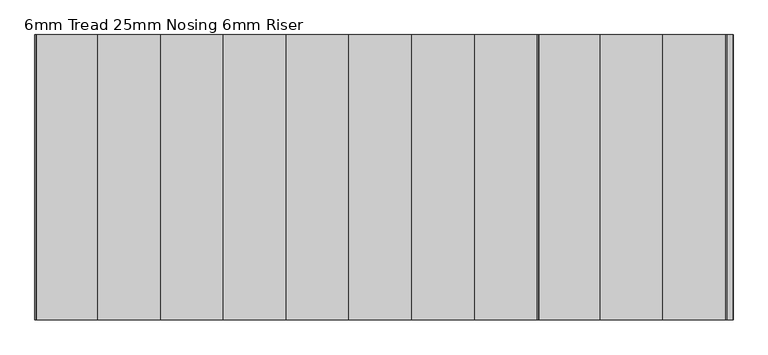
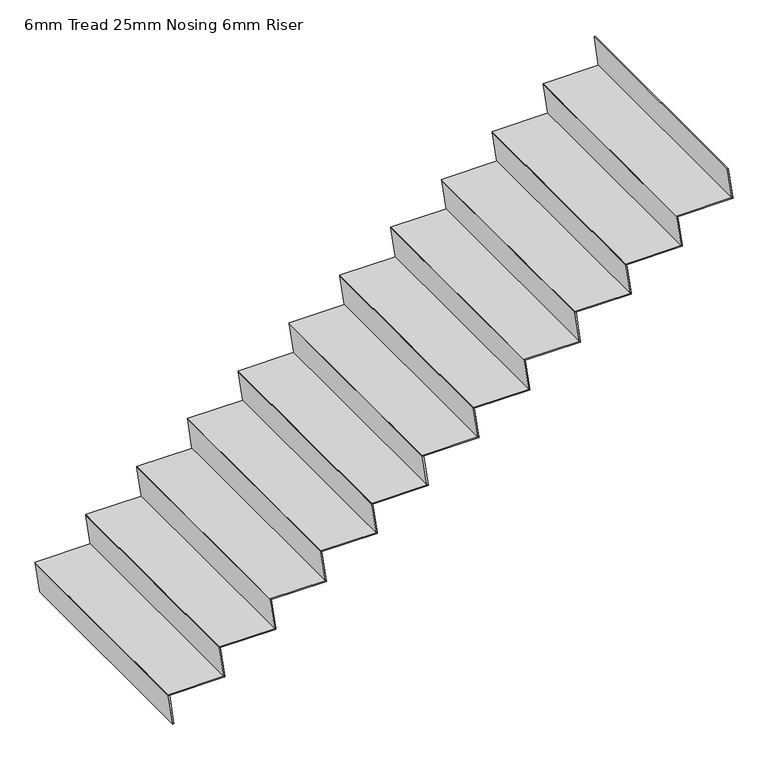
"""IFC4 building model written with IfcOpenShell, lengths in millimetres: stair flight geometry, 6mm Tread 25mm Nosing 6mm Riser."""

from ifc_helpers import new_model, si_unit, frame, origin, place, context, project, spatial, polyline, outline, extrude, source, transform, mapped, element, save


def stair_flight_6mm_tread_25mm_nosing_6mm_riser_570a7bc1(model_context):
    return source(origin(), model_context, "Body", "SweptSolid", [
        extrude(outline(polyline([(4266.6666667, 13631.0590357), (4266.6666667, 13325.0), (4260.6666667, 13325.84375), (4260.6666667, 13631.9027857), (4266.6666667, 13631.0590357)])), frame((0.0, 10220.4345331, 0.0), z_axis=(0.0, 1.0, 0.0), x_axis=(0.0, 0.0, 1.0)), (0.0, 0.0, 1.0), 1250.0),
        extrude(outline(polyline([(4260.6666667, 13325.84375), (4088.8888889, 13350.0), (4088.8888889, 13356.0590357), (4260.6666667, 13331.9027857), (4260.6666667, 13325.84375)])), frame((0.0, 10220.4345331, 0.0), z_axis=(0.0, 1.0, 0.0), x_axis=(0.0, 0.0, 1.0)), (0.0, 0.0, 1.0), 1250.0),
        extrude(outline(polyline([(4438.4444444, 13600.84375), (4266.6666667, 13625.0), (4266.6666667, 13631.0590357), (4438.4444444, 13606.9027857), (4438.4444444, 13600.84375)])), frame((0.0, 10220.4345331, 0.0), z_axis=(0.0, 1.0, 0.0), x_axis=(0.0, 0.0, 1.0)), (0.0, 0.0, 1.0), 1250.0),
        extrude(outline(polyline([(4444.4444444, 13906.0590357), (4444.4444444, 13600.0), (4438.4444444, 13600.84375), (4438.4444444, 13906.9027857), (4444.4444444, 13906.0590357)])), frame((0.0, 10220.4345331, 0.0), z_axis=(0.0, 1.0, 0.0), x_axis=(0.0, 0.0, 1.0)), (0.0, 0.0, 1.0), 1250.0),
        extrude(outline(polyline([(4616.2222222, 13875.84375), (4444.4444444, 13900.0), (4444.4444444, 13906.0590357), (4616.2222222, 13881.9027857), (4616.2222222, 13875.84375)])), frame((0.0, 10220.4345331, 0.0), z_axis=(0.0, 1.0, 0.0), x_axis=(0.0, 0.0, 1.0)), (0.0, 0.0, 1.0), 1250.0),
        extrude(outline(polyline([(4622.2222222, 14181.0590357), (4622.2222222, 13875.0), (4616.2222222, 13875.84375), (4616.2222222, 14181.9027857), (4622.2222222, 14181.0590357)])), frame((0.0, 10220.4345331, 0.0), z_axis=(0.0, 1.0, 0.0), x_axis=(0.0, 0.0, 1.0)), (0.0, 0.0, 1.0), 1250.0),
        extrude(outline(polyline([(4794.0, 14150.84375), (4622.2222222, 14175.0), (4622.2222222, 14181.0590357), (4794.0, 14156.9027857), (4794.0, 14150.84375)])), frame((0.0, 10220.4345331, 0.0), z_axis=(0.0, 1.0, 0.0), x_axis=(0.0, 0.0, 1.0)), (0.0, 0.0, 1.0), 1250.0),
        extrude(outline(polyline([(4800.0, 14456.0590357), (4800.0, 14150.0), (4794.0, 14150.84375), (4794.0, 14456.9027857), (4800.0, 14456.0590357)])), frame((0.0, 10220.4345331, 0.0), z_axis=(0.0, 1.0, 0.0), x_axis=(0.0, 0.0, 1.0)), (0.0, 0.0, 1.0), 1250.0),
        extrude(outline(polyline([(4971.7777778, 14425.84375), (4800.0, 14450.0), (4800.0, 14456.0590357), (4971.7777778, 14431.9027857), (4971.7777778, 14425.84375)])), frame((0.0, 10220.4345331, 0.0), z_axis=(0.0, 1.0, 0.0), x_axis=(0.0, 0.0, 1.0)), (0.0, 0.0, 1.0), 1250.0),
        extrude(outline(polyline([(4977.7777778, 14731.0590357), (4977.7777778, 14425.0), (4971.7777778, 14425.84375), (4971.7777778, 14731.9027857), (4977.7777778, 14731.0590357)])), frame((0.0, 10220.4345331, 0.0), z_axis=(0.0, 1.0, 0.0), x_axis=(0.0, 0.0, 1.0)), (0.0, 0.0, 1.0), 1250.0),
        extrude(outline(polyline([(5149.5555556, 14700.84375), (4977.7777778, 14725.0), (4977.7777778, 14731.0590357), (5149.5555556, 14706.9027857), (5149.5555556, 14700.84375)])), frame((0.0, 10220.4345331, 0.0), z_axis=(0.0, 1.0, 0.0), x_axis=(0.0, 0.0, 1.0)), (0.0, 0.0, 1.0), 1250.0),
        extrude(outline(polyline([(5155.5555556, 15006.0590357), (5155.5555556, 14700.0), (5149.5555556, 14700.84375), (5149.5555556, 15006.9027857), (5155.5555556, 15006.0590357)])), frame((0.0, 10220.4345331, 0.0), z_axis=(0.0, 1.0, 0.0), x_axis=(0.0, 0.0, 1.0)), (0.0, 0.0, 1.0), 1250.0),
        extrude(outline(polyline([(5327.3333333, 14975.84375), (5155.5555556, 15000.0), (5155.5555556, 15006.0590357), (5327.3333333, 14981.9027857), (5327.3333333, 14975.84375)])), frame((0.0, 10220.4345331, 0.0), z_axis=(0.0, 1.0, 0.0), x_axis=(0.0, 0.0, 1.0)), (0.0, 0.0, 1.0), 1250.0),
        extrude(outline(polyline([(5333.3333333, 15281.0590357), (5333.3333333, 14975.0), (5327.3333333, 14975.84375), (5327.3333333, 15281.9027857), (5333.3333333, 15281.0590357)])), frame((0.0, 10220.4345331, 0.0), z_axis=(0.0, 1.0, 0.0), x_axis=(0.0, 0.0, 1.0)), (0.0, 0.0, 1.0), 1250.0),
        extrude(outline(polyline([(5505.1111111, 15250.84375), (5333.3333333, 15275.0), (5333.3333333, 15281.0590357), (5505.1111111, 15256.9027857), (5505.1111111, 15250.84375)])), frame((0.0, 10220.4345331, 0.0), z_axis=(0.0, 1.0, 0.0), x_axis=(0.0, 0.0, 1.0)), (0.0, 0.0, 1.0), 1250.0),
        extrude(outline(polyline([(5511.1111111, 15556.0590357), (5511.1111111, 15250.0), (5505.1111111, 15250.84375), (5505.1111111, 15556.9027857), (5511.1111111, 15556.0590357)])), frame((0.0, 10220.4345331, 0.0), z_axis=(0.0, 1.0, 0.0), x_axis=(0.0, 0.0, 1.0)), (0.0, 0.0, 1.0), 1250.0),
        extrude(outline(polyline([(5682.8888889, 15525.84375), (5511.1111111, 15550.0), (5511.1111111, 15556.0590357), (5682.8888889, 15531.9027857), (5682.8888889, 15525.84375)])), frame((0.0, 10220.4345331, 0.0), z_axis=(0.0, 1.0, 0.0), x_axis=(0.0, 0.0, 1.0)), (0.0, 0.0, 1.0), 1250.0),
        extrude(outline(polyline([(5688.8888889, 15831.0590357), (5688.8888889, 15525.0), (5682.8888889, 15525.84375), (5682.8888889, 15831.9027857), (5688.8888889, 15831.0590357)])), frame((0.0, 10220.4345331, 0.0), z_axis=(0.0, 1.0, 0.0), x_axis=(0.0, 0.0, 1.0)), (0.0, 0.0, 1.0), 1250.0),
        extrude(outline(polyline([(5860.6666667, 15800.84375), (5688.8888889, 15825.0), (5688.8888889, 15831.0590357), (5860.6666667, 15806.9027857), (5860.6666667, 15800.84375)])), frame((0.0, 10220.4345331, 0.0), z_axis=(0.0, 1.0, 0.0), x_axis=(0.0, 0.0, 1.0)), (0.0, 0.0, 1.0), 1250.0),
        extrude(outline(polyline([(5866.6666667, 16106.0590357), (5866.6666667, 15800.0), (5860.6666667, 15800.84375), (5860.6666667, 16106.9027857), (5866.6666667, 16106.0590357)])), frame((0.0, 10220.4345331, 0.0), z_axis=(0.0, 1.0, 0.0), x_axis=(0.0, 0.0, 1.0)), (0.0, 0.0, 1.0), 1250.0),
        extrude(outline(polyline([(6038.4444444, 16075.84375), (5866.6666667, 16100.0), (5866.6666667, 16106.0590357), (6038.4444444, 16081.9027857), (6038.4444444, 16075.84375)])), frame((0.0, 10220.4345331, 0.0), z_axis=(0.0, 1.0, 0.0), x_axis=(0.0, 0.0, 1.0)), (0.0, 0.0, 1.0), 1250.0),
        extrude(outline(polyline([(6216.2222222, 16350.84375), (6044.4444444, 16375.0), (6044.4444444, 16381.0590357), (6216.2222222, 16356.9027857), (6216.2222222, 16350.84375)])), frame((0.0, 10220.4345331, 0.0), z_axis=(0.0, 1.0, 0.0), x_axis=(0.0, 0.0, 1.0)), (0.0, 0.0, 1.0), 1250.0),
        extrude(outline(polyline([(6044.4444444, 16381.0590357), (6044.4444444, 16075.0), (6038.4444444, 16075.84375), (6038.4444444, 16381.9027857), (6044.4444444, 16381.0590357)])), frame((0.0, 10220.4345331, 0.0), z_axis=(0.0, 1.0, 0.0), x_axis=(0.0, 0.0, 1.0)), (0.0, 0.0, 1.0), 1250.0),
    ])


if __name__ == "__main__":
    model = new_model("IFC4")
    model_context = context("Model", 3, world=origin())
    ifc_project = project(units=[si_unit("LENGTHUNIT", "METRE", prefix="MILLI")], contexts=[model_context])
    site = spatial("IfcSite", under=ifc_project)
    building = spatial("IfcBuilding", under=site)
    placement = place(None, origin())
    stair_flight_6mm_tread_25mm_nosing_6mm_riser_shape = stair_flight_6mm_tread_25mm_nosing_6mm_riser_570a7bc1(model_context)
    element("IfcStairFlight", 1, ObjectType="6mm Tread 25mm Nosing 6mm Riser", at=placement, inside=building, context=model_context, shape_type="MappedRepresentation", body=[
        mapped(stair_flight_6mm_tread_25mm_nosing_6mm_riser_shape, transform((0.0, 0.0, 0.0), x_axis=(1.0, 0.0, 0.0), y_axis=(0.0, 1.0, 0.0), z_axis=(0.0, 0.0, 1.0))),
    ])
    save(model, "model.ifc")

# Revit data of these elements
# Element 1 (IfcStairFlight, "6mm Tread 25mm Nosing 6mm Riser")
#   Materials on its faces: "Steel, Paint Finish, Dark Gray"
# Materials
#   "Steel, Paint Finish, Dark Gray": class "Metal", colour RGB 89 89 89, transparency 0, Description = "Steel, paint finish, dark gray, glossy", Cost = 0
